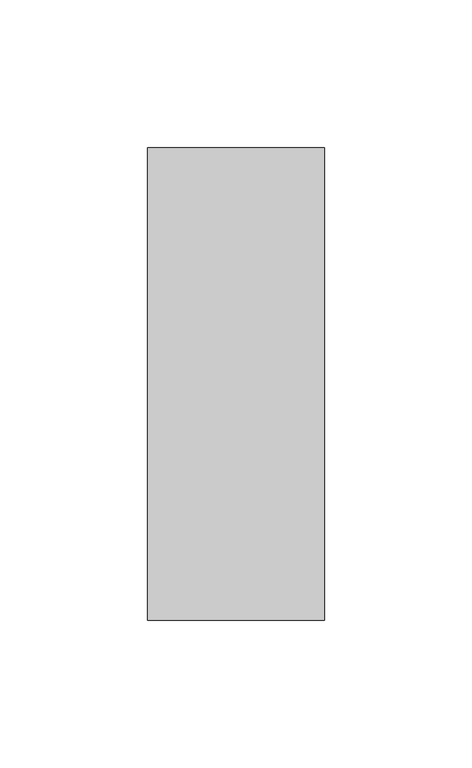
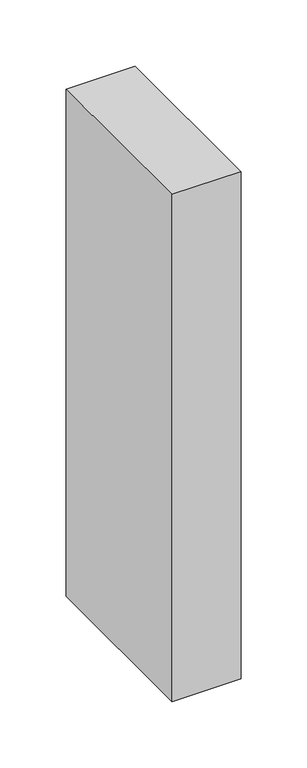
"""IFC4 building model written with IfcOpenShell, lengths in millimetres: column geometry, Madeira de lei-Coluna : Pontalete 6X16cm."""

import ifcopenshell
import ifcopenshell.guid

model = None  # the IFC model being written
_history = None  # IfcOwnerHistory: only IFC2X3 demands one
_inside = {}  # id of a spatial element -> (the spatial element, [elements in it])
_under = {}  # id of a project, library or spatial element -> (it, [spatial elements below it])
_declared = {}  # id of a project -> (the project, [libraries it declares])
_typed = {}  # id of a type object -> (the type object, [elements of that type])
_made_of = {}  # id of a material, layer set ... -> (it, [elements and type objects made of it])


def new_model(schema):
    """Start an empty IFC model of exactly this schema.

    Asked for "IFC4X3", IfcOpenShell would pick the latest addendum, in which some entities
    have other attributes; the version numbers below select the first issue.
    IFC2X3 requires an IfcOwnerHistory on every rooted entity: one is made here for all.
    """
    global model, _history
    if schema == "IFC4X3":
        model = ifcopenshell.file(schema_version=(4, 3, 0, 0))
    else:
        model = ifcopenshell.file(schema=schema)
    _inside.clear()
    _under.clear()
    _declared.clear()
    _typed.clear()
    _made_of.clear()
    _history = None
    if model.schema == "IFC2X3":
        org = make("IfcOrganization", Name="unknown")
        user = make(
            "IfcPersonAndOrganization",
            ThePerson=make("IfcPerson", FamilyName="unknown"),
            TheOrganization=org,
        )
        app = make(
            "IfcApplication",
            ApplicationDeveloper=org,
            Version="unknown",
            ApplicationFullName="unknown",
            ApplicationIdentifier="unknown",
        )
        _history = make(
            "IfcOwnerHistory",
            OwningUser=user,
            OwningApplication=app,
            ChangeAction="ADDED",
            CreationDate=0,
        )
    return model


def make(cls, **values):
    """One entity of the class cls with the attributes given. An attribute that is None is left unset."""
    return model.create_entity(
        cls, **{name: value for name, value in values.items() if value is not None}
    )


def rooted(cls, **values):
    """An entity with a GlobalId (a new one), such as an element, a storey or a relation."""
    return make(cls, GlobalId=ifcopenshell.guid.new(), OwnerHistory=_history, **values)


def si_unit(unit_type, name, prefix=None):
    """IfcSIUnit, for example si_unit("LENGTHUNIT", "METRE", prefix="MILLI")."""
    return make("IfcSIUnit", UnitType=unit_type, Prefix=prefix, Name=name)


def assignment(units):
    """IfcUnitAssignment: the units of a project."""
    return None if units is None else make("IfcUnitAssignment", Units=units)


def point(xyz):
    """IfcCartesianPoint."""
    return None if xyz is None else make("IfcCartesianPoint", Coordinates=xyz)


def direction(xyz):
    """IfcDirection."""
    return None if xyz is None else make("IfcDirection", DirectionRatios=xyz)


def frame(location, z_axis=None, x_axis=None):
    """IfcAxis2Placement3D, a coordinate frame: its origin and axes. An axis left out is left unset."""
    return make(
        "IfcAxis2Placement3D",
        Location=point(location),
        Axis=direction(z_axis),
        RefDirection=direction(x_axis),
    )


def origin():
    """The frame at (0, 0, 0) with its axes left unset."""
    return frame((0.0, 0.0, 0.0))


def place(relative_to, where):
    """IfcLocalPlacement: puts the frame where relative to a parent placement (None: the world)."""
    return make(
        "IfcLocalPlacement", PlacementRelTo=relative_to, RelativePlacement=where
    )


def context(
    kind, dimensions, precision=None, world=None, true_north=None, identifier=None
):
    """IfcGeometricRepresentationContext, for example the 3D "Model" context."""
    return make(
        "IfcGeometricRepresentationContext",
        ContextIdentifier=identifier,
        ContextType=kind,
        CoordinateSpaceDimension=dimensions,
        Precision=precision,
        WorldCoordinateSystem=world,
        TrueNorth=true_north,
    )


def project(units=None, contexts=None):
    """IfcProject with its units and contexts."""
    return rooted(
        "IfcProject",
        Name="project",
        RepresentationContexts=contexts,
        UnitsInContext=assignment(units),
    )


def spatial(cls, under=None, at=None, **own):
    """A site, building, storey or space (cls), placed at a placement, below another one or the project."""
    s = rooted(cls, ObjectPlacement=at, **own)
    if under is not None:
        _under.setdefault(under.id(), (under, []))[1].append(s)
    return s


def polyline(points):
    """IfcPolyline through the points."""
    return make("IfcPolyline", Points=[point(p) for p in points])


def outline(outer, holes=None, kind="AREA"):
    """IfcArbitraryClosedProfileDef: a profile drawn as a closed curve; with holes, ...WithVoids."""
    if holes is None:
        return make("IfcArbitraryClosedProfileDef", ProfileType=kind, OuterCurve=outer)
    return make(
        "IfcArbitraryProfileDefWithVoids",
        ProfileType=kind,
        OuterCurve=outer,
        InnerCurves=holes,
    )


def extrude(swept, where, along, depth):
    """IfcExtrudedAreaSolid: the profile swept, set in the frame where, extruded along a direction by depth."""
    return make(
        "IfcExtrudedAreaSolid",
        SweptArea=swept,
        Position=where,
        ExtrudedDirection=direction(along),
        Depth=depth,
    )


def shape(context_of_items, identifier, shape_type, items):
    """IfcShapeRepresentation: the items that make up one representation, for example the "Body"."""
    return make(
        "IfcShapeRepresentation",
        ContextOfItems=context_of_items,
        RepresentationIdentifier=identifier,
        RepresentationType=shape_type,
        Items=items,
    )


def source(mapping_origin, context_of_items, identifier, shape_type, items):
    """IfcRepresentationMap: a shape defined once, which mapped items show again and again."""
    return make(
        "IfcRepresentationMap",
        MappingOrigin=mapping_origin,
        MappedRepresentation=shape(context_of_items, identifier, shape_type, items),
    )


def transform(
    local_origin,
    x_axis=None,
    y_axis=None,
    z_axis=None,
    scale=None,
    scale2=None,
    scale3=None,
    uniform=True,
):
    """IfcCartesianTransformationOperator3D, or its non-uniform kind. x_axis, y_axis, z_axis: its Axis1, 2, 3."""
    if uniform:
        return make(
            "IfcCartesianTransformationOperator3D",
            Axis1=direction(x_axis),
            Axis2=direction(y_axis),
            LocalOrigin=point(local_origin),
            Scale=scale,
            Axis3=direction(z_axis),
        )
    return make(
        "IfcCartesianTransformationOperator3DnonUniform",
        Axis1=direction(x_axis),
        Axis2=direction(y_axis),
        LocalOrigin=point(local_origin),
        Scale=scale,
        Axis3=direction(z_axis),
        Scale2=scale2,
        Scale3=scale3,
    )


def mapped(mapping_source, mapping_target):
    """IfcMappedItem: shows the shape of a source again, moved by a transform."""
    return make(
        "IfcMappedItem", MappingSource=mapping_source, MappingTarget=mapping_target
    )


def made_of(thing, what):
    """Note that an element or type object is made of a material, layer set ...; save() writes the relation."""
    if what is not None:
        _made_of.setdefault(what.id(), (what, []))[1].append(thing)
    return thing


def element(
    cls,
    number,
    at=None,
    inside=None,
    cuts=None,
    type_object=None,
    material=None,
    context=None,
    identifier="Body",
    shape_type=None,
    held_by="IfcProductDefinitionShape",
    body=None,
    shapes=None,
    **own,
):
    """One element of the class cls, such as IfcWall. Its Tag is "e" and its number.

    at: its placement. inside: the storey or other place that contains it. cuts: it is an
    opening in that element (IfcRelVoidsElement). A single representation is given by context,
    identifier, shape_type and body (its items); several are given by shapes. held_by: the class
    of the entity that holds the representations. save() writes the other relations.
    """
    e = rooted(cls, Tag="e%d" % number, ObjectPlacement=at, **own)
    if body is not None:
        shapes = [shape(context, identifier, shape_type, body)]
    if shapes is not None:
        e.Representation = make(held_by, Representations=shapes)
    if inside is not None:
        _inside.setdefault(inside.id(), (inside, []))[1].append(e)
    if cuts is not None:
        rooted(
            "IfcRelVoidsElement", RelatingBuildingElement=cuts, RelatedOpeningElement=e
        )
    if type_object is not None:
        _typed.setdefault(type_object.id(), (type_object, []))[1].append(e)
    return made_of(e, material)


def aggregate(whole, parts):
    """IfcRelAggregates: a whole, such as a stair, and the parts it consists of."""
    return rooted("IfcRelAggregates", RelatingObject=whole, RelatedObjects=parts)


def save(model, path):
    """Write the relations noted so far, then the file.

    IfcRelAggregates (storeys below a building ...), IfcRelContainedInSpatialStructure (elements
    in a storey), IfcRelDefinesByType, IfcRelAssociatesMaterial and IfcRelDeclares: one each for
    every whole, place, type object, material and project.
    """
    for whole, parts in _under.values():
        aggregate(whole, parts)
    for where, things in _inside.values():
        rooted(
            "IfcRelContainedInSpatialStructure",
            RelatedElements=things,
            RelatingStructure=where,
        )
    for kind, things in _typed.values():
        rooted("IfcRelDefinesByType", RelatedObjects=things, RelatingType=kind)
    for what, things in _made_of.values():
        rooted("IfcRelAssociatesMaterial", RelatedObjects=things, RelatingMaterial=what)
    for by, libraries in _declared.values():
        rooted("IfcRelDeclares", RelatingContext=by, RelatedDefinitions=libraries)
    model.write(path)


def column_6c15bf79(model_context):
    return source(origin(), model_context, "Body", "SweptSolid", [
        extrude(outline(polyline([(30.0, 80.0), (30.0, -80.0), (-30.0, -80.0), (-30.0, 80.0), (30.0, 80.0)])), frame((0.0, 0.0, 6710.0), z_axis=(0.0, 0.0, 1.0), x_axis=(1.0, 0.0, 0.0)), (0.0, 0.0, 1.0), 467.5),
    ])


if __name__ == "__main__":
    model = new_model("IFC4")
    model_context = context("Model", 3, world=origin())
    ifc_project = project(units=[si_unit("LENGTHUNIT", "METRE", prefix="MILLI")], contexts=[model_context])
    site = spatial("IfcSite", under=ifc_project)
    building = spatial("IfcBuilding", under=site)
    placement = place(None, origin())
    column_shape = column_6c15bf79(model_context)
    element("IfcColumn", 1, ObjectType="Madeira de lei-Coluna : Pontalete 6X16cm", at=placement, inside=building, context=model_context, shape_type="MappedRepresentation", body=[
        mapped(column_shape, transform((0.0, 0.0, 0.0), x_axis=(1.0, 0.0, 0.0), y_axis=(0.0, 1.0, 0.0), z_axis=(0.0, 0.0, 1.0))),
    ])
    save(model, "model.ifc")

# Revit data of these elements
# Type "Madeira de lei-Coluna : Pontalete 6X16cm"
#   A = 0.01952 m²
#   b = 0.06 m
#   d = 0.16 m
#   Structural Material [instance default] = none
#   Assembly Code = ""
# Element 1 (IfcColumn, "Madeira de lei-Coluna : Pontalete 6X16cm")
#   Structural Material = .MADEIRAMENTO
#   Materials on its faces: ".MADEIRAMENTO"
# Materials
#   ".MADEIRAMENTO": class ".CC_MADEIRAS", colour RGB 212 179 113, transparency 0, Cost = 0
